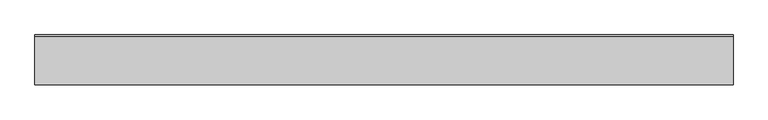
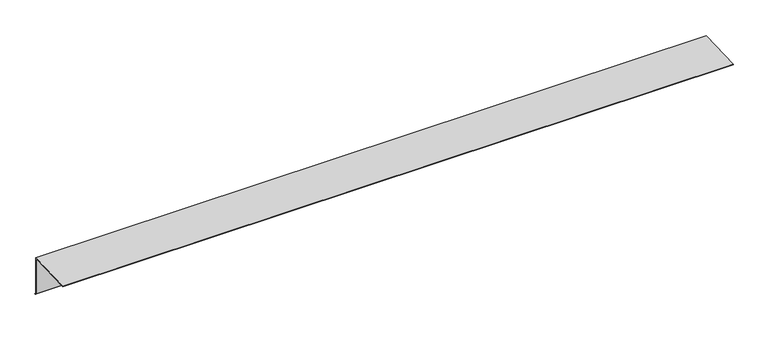
"""IFC4 building model written with IfcOpenShell, lengths in millimetres: proxy geometry, Generic Models 7:Generic Models 1:337419:Generic Models 1:337419 : Generic Models 7:Generic Models 1:337419:24 : Generic Models 7:Generic Models 1:337419:Generic Models 1:337419 : Generic Models 7:Generic Models 1:337419:301336."""

from ifc_helpers import new_model, si_unit, frame, origin, place, context, project, spatial, polyline, outline, extrude, source, transform, mapped, element, save


def generic_models_b1bffb81(model_context):
    return source(origin(), model_context, "Body", "SweptSolid", [
        extrude(outline(polyline([(-536826.9607982, 10233.5704633), (-536827.0764531, 10236.3461799), (-536491.2329484, 10250.3396593), (-536491.2329484, 9979.4031787), (-536477.7625642, 9965.9327946), (-536479.7269953, 9963.9683635), (-536494.0110734, 9978.2524417), (-536494.0110734, 10247.4433685), (-536826.9607982, 10233.5704633)])), frame((591306.0367242, 0.0, 0.0), z_axis=(1.0, 0.0, 0.0), x_axis=(0.0, 1.0, 0.0)), (0.0, 0.0, 1.0), 4876.8),
    ])


if __name__ == "__main__":
    model = new_model("IFC4")
    model_context = context("Model", 3, world=origin())
    ifc_project = project(units=[si_unit("LENGTHUNIT", "METRE", prefix="MILLI")], contexts=[model_context])
    site = spatial("IfcSite", under=ifc_project)
    building = spatial("IfcBuilding", under=site)
    placement = place(None, origin())
    generic_models_shape = generic_models_b1bffb81(model_context)
    element("IfcBuildingElementProxy", 1, Name="Generic Models 7:Generic Models 1:337419:Generic Models 1:337419 : Generic Models 7:Generic Models 1:337419:24 : Generic Models 7:Generic Models 1:337419:Generic Models 1:337419 : Generic Models 7:Generic Models 1:337419:301336", ObjectType="Generic Models 7:Generic Models 1:337419:Generic Models 1:337419 : Generic Models 7:Generic Models 1:337419:24 : Generic Models 7:Generic Models 1:337419:Generic Models 1:337419 : Generic Models 7:Generic Models 1:337419:301336", at=placement, inside=building, context=model_context, shape_type="MappedRepresentation", body=[
        mapped(generic_models_shape, transform((0.0, 0.0, 0.0), x_axis=(1.0, 0.0, 0.0), y_axis=(0.0, 1.0, 0.0), z_axis=(0.0, 0.0, 1.0))),
    ])
    save(model, "model.ifc")

# Revit data of these elements
# Type "Generic Models 7:Generic Models 1:337419:Generic Models 1:337419 : Generic Models 7:Generic Models 1:337419:24 : Generic Models 7:Generic Models 1:337419:Generic Models 1:337419 : Generic Models 7:Generic Models 1:337419:301336"
#   NameOverride = "Generic Models 7:Generic Models 1:337419:Generic Models 1:337419 : Generic Models 7:Generic Models 1:337419:301336"
#   ObjectTypeOverride = "Generic Models 1:337419 : Generic Models 7:Generic Models 1:337419"
#   Reference = "Generic Models 1"
#   Tag = "301336"
# Element 1 (IfcBuildingElementProxy, "Generic Models 7:Generic Models 1:337419:Generic Models 1:337419 : Generic Models 7:Generic Models 1:337419:24 : Generic Models 7:Generic Models 1:337419:Generic Models 1:337419 : Generic Models 7:Generic Models 1:337419:301336")
#   Materials on its faces: "BOX HIGH SIDE EAVE TRIM (FL-33)"
# Materials
#   "BOX HIGH SIDE EAVE TRIM (FL-33)": class "Generic", colour RGB 182 182 182, transparency 0, Cost = 0
